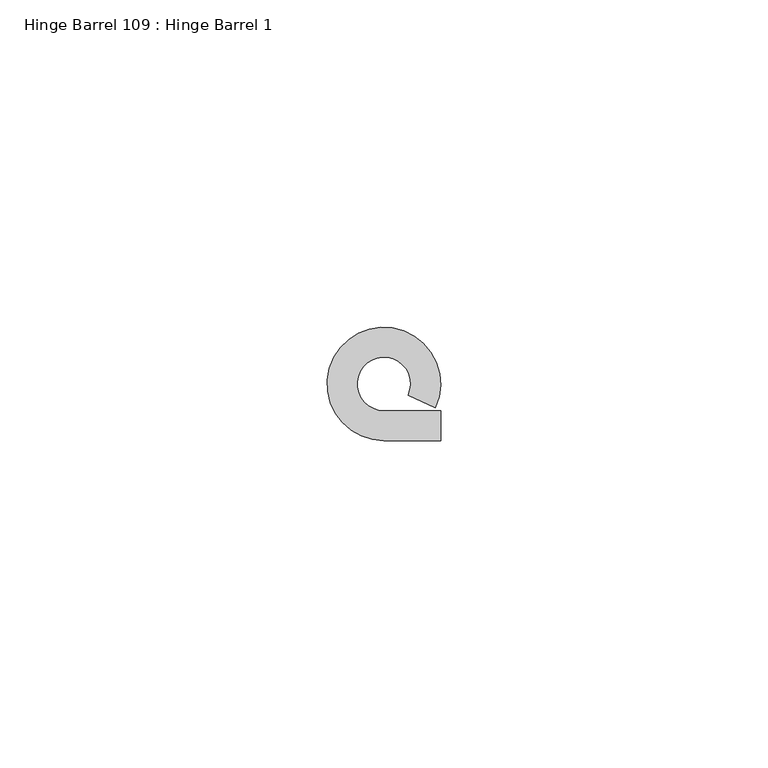
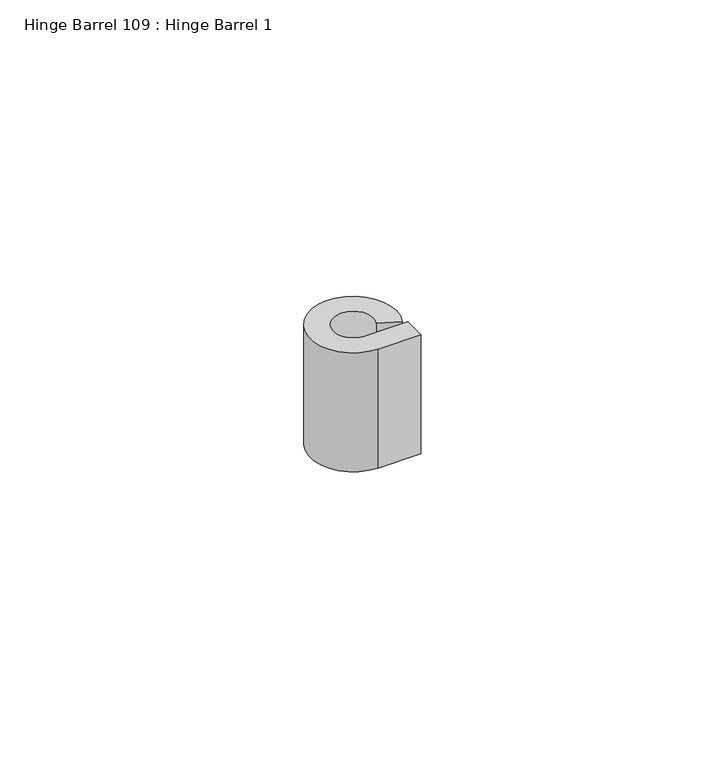
"""IFC4 building model written with IfcOpenShell, lengths in millimetres: proxy geometry, Hinge Barrel 109 : Hinge Barrel 1."""

from ifc_helpers import new_model, si_unit, point, frame, frame_2d, origin, place, context, project, spatial, polyline, circle_curve, trimmed, segment, composite_curve, outline, extrude, source, transform, mapped, element, save


def hinge_barrel_109_hinge_barrel_1_58d778a9(model_context):
    return source(origin(), model_context, "Body", "SweptSolid", [
        extrude(outline(composite_curve([segment(polyline([(587323.2214739, -534104.7943841), (587327.7934739, -534104.7943841), (587327.7934739, -534109.3584466), (587319.1320739, -534109.3584466)]), True, "CONTINUOUS"), segment(trimmed(circle_curve(frame_2d((587319.1320739, -534100.7049841)), 8.6534625), [point((587319.1320739, -534109.3584466))], [point((587326.986084, -534104.3377433))], False, "CARTESIAN"), True, "CONTINUOUS"), segment(polyline([(587326.986084, -534104.3377433), (587322.8436736, -534102.421731)]), True, "CONTINUOUS"), segment(trimmed(circle_curve(frame_2d((587319.1320739, -534100.7049841)), 4.0894), [point((587322.8436736, -534102.421731))], [point((587319.1320739, -534104.7943841))], True, "CARTESIAN"), True, "CONTINUOUS"), segment(polyline([(587319.1320739, -534104.7943841), (587323.2214739, -534104.7943841)]), True, "CONTINUOUS")], self_intersect=False)), frame((0.0, 0.0, 311.15), z_axis=(0.0, 0.0, 1.0), x_axis=(1.0, 0.0, 0.0)), (0.0, 0.0, 1.0), 25.4),
    ])


if __name__ == "__main__":
    model = new_model("IFC4")
    model_context = context("Model", 3, world=origin())
    ifc_project = project(units=[si_unit("LENGTHUNIT", "METRE", prefix="MILLI")], contexts=[model_context])
    site = spatial("IfcSite", under=ifc_project)
    building = spatial("IfcBuilding", under=site)
    placement = place(None, origin())
    hinge_barrel_109_hinge_barrel_1_shape = hinge_barrel_109_hinge_barrel_1_58d778a9(model_context)
    element("IfcBuildingElementProxy", 1, Name="Hinge Barrel 109 : Hinge Barrel 1", ObjectType="Hinge Barrel 109 : Hinge Barrel 1", at=placement, inside=building, context=model_context, shape_type="MappedRepresentation", body=[
        mapped(hinge_barrel_109_hinge_barrel_1_shape, transform((0.0, 0.0, 0.0), x_axis=(1.0, 0.0, 0.0), y_axis=(0.0, 1.0, 0.0), z_axis=(0.0, 0.0, 1.0))),
    ])
    save(model, "model.ifc")

# Revit data of these elements
# Element 1 (IfcBuildingElementProxy, "Hinge Barrel 109 : Hinge Barrel 1")
#   Materials on its faces: "6\"X6\" WELD-ON STL BUTT HINGE"
# Materials
#   "6\"X6\" WELD-ON STL BUTT HINGE": class "Metal", colour RGB 189 187 185, transparency 0, Description = "Carbon steel", Cost = 0
